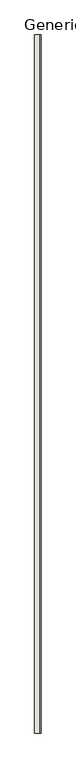
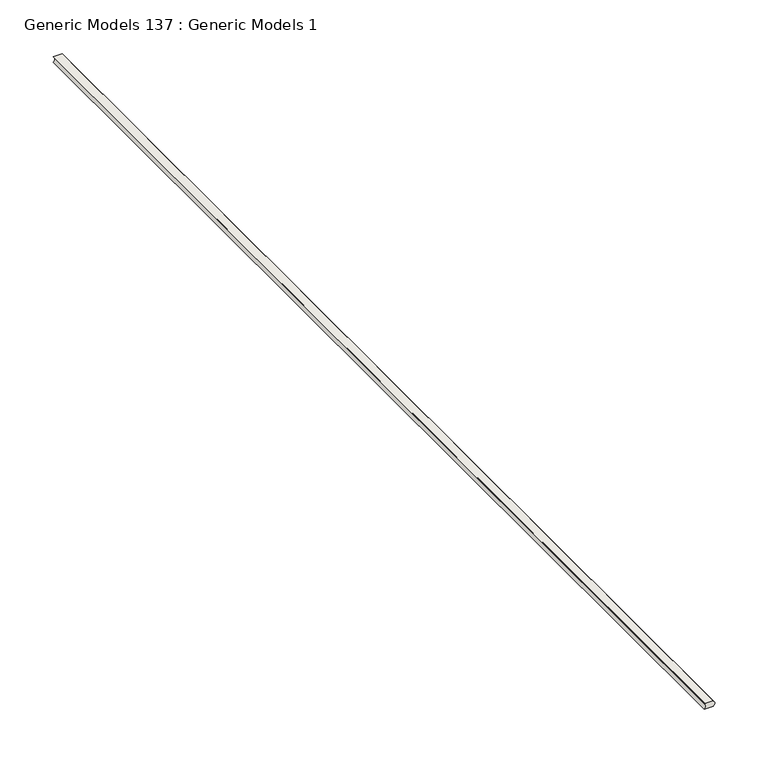
"""IFC4 building model written with IfcOpenShell, lengths in millimetres: wall geometry, Generic Models 137 : Generic Models 1."""

from ifc_helpers import new_model, si_unit, point, frame, frame_2d, origin, place, context, project, spatial, polyline, circle_curve, trimmed, segment, composite_curve, outline, extrude, source, transform, mapped, element, save


def generic_models_137_generic_models_1_b98dbe0e(model_context):
    return source(origin(), model_context, "Body", "SweptSolid", [
        extrude(outline(composite_curve([segment(polyline([(0.0, 50900.0125), (0.0, 50909.5375)]), True, "CONTINUOUS"), segment(trimmed(circle_curve(frame_2d((3.175, 50906.6227595)), 4.3100275), [point((0.0, 50909.5375))], [point((6.35, 50909.5375))], False, "CARTESIAN"), True, "CONTINUOUS"), segment(polyline([(6.35, 50909.5375), (6.35, 50900.0125)]), True, "CONTINUOUS"), segment(trimmed(circle_curve(frame_2d((3.175, 50897.0977595)), 4.3100275), [point((6.35, 50900.0125))], [point((0.0, 50900.0125))], True, "CARTESIAN"), True, "CONTINUOUS")], self_intersect=False)), frame((0.0, 0.0, 0.0), z_axis=(0.0, 1.0, 0.0), x_axis=(0.0, 0.0, 1.0)), (0.0, 0.0, 1.0), 1219.2),
    ])


if __name__ == "__main__":
    model = new_model("IFC4")
    model_context = context("Model", 3, world=origin())
    ifc_project = project(units=[si_unit("LENGTHUNIT", "METRE", prefix="MILLI")], contexts=[model_context])
    site = spatial("IfcSite", under=ifc_project)
    building = spatial("IfcBuilding", under=site)
    placement = place(None, origin())
    generic_models_137_generic_models_1_shape = generic_models_137_generic_models_1_b98dbe0e(model_context)
    element("IfcWall", 1, ObjectType="Generic Models 137 : Generic Models 1", at=placement, inside=building, context=model_context, shape_type="MappedRepresentation", body=[
        mapped(generic_models_137_generic_models_1_shape, transform((0.0, 0.0, 0.0), x_axis=(1.0, 0.0, 0.0), y_axis=(0.0, 1.0, 0.0), z_axis=(0.0, 0.0, 1.0))),
    ])
    save(model, "model.ifc")

# Revit data of these elements
# Element 1 (IfcWall, "Generic Models 137 : Generic Models 1")
#   Materials on its faces: "SEALANT (W/ BACKER ROD IF NECESSARY)"
# Materials
#   "SEALANT (W/ BACKER ROD IF NECESSARY)": class "Unassigned", colour RGB 120 120 120, transparency 0, Cost = 0
